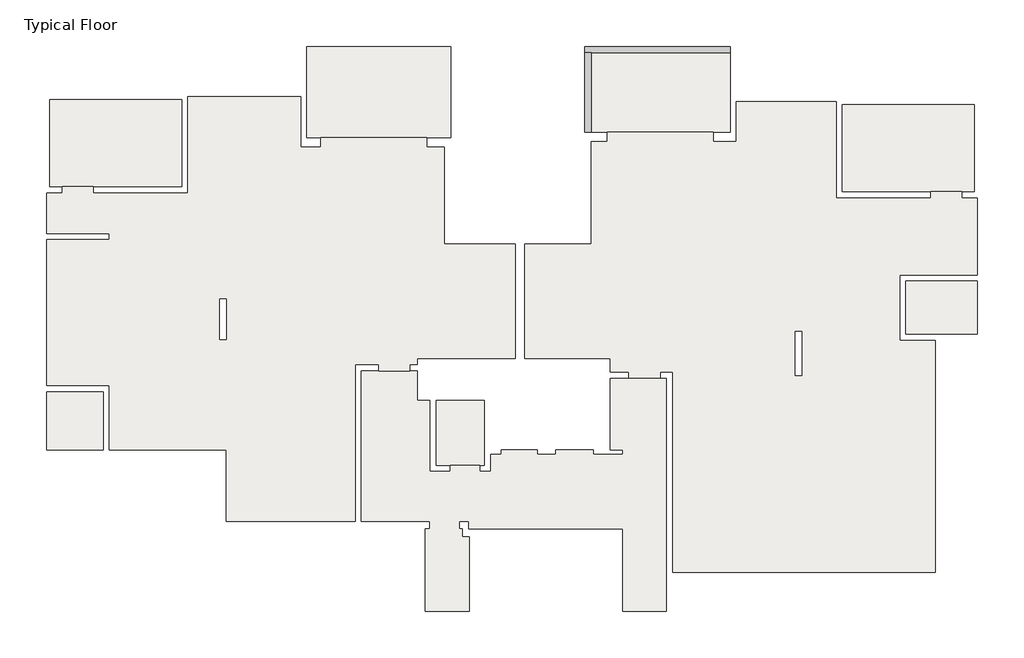
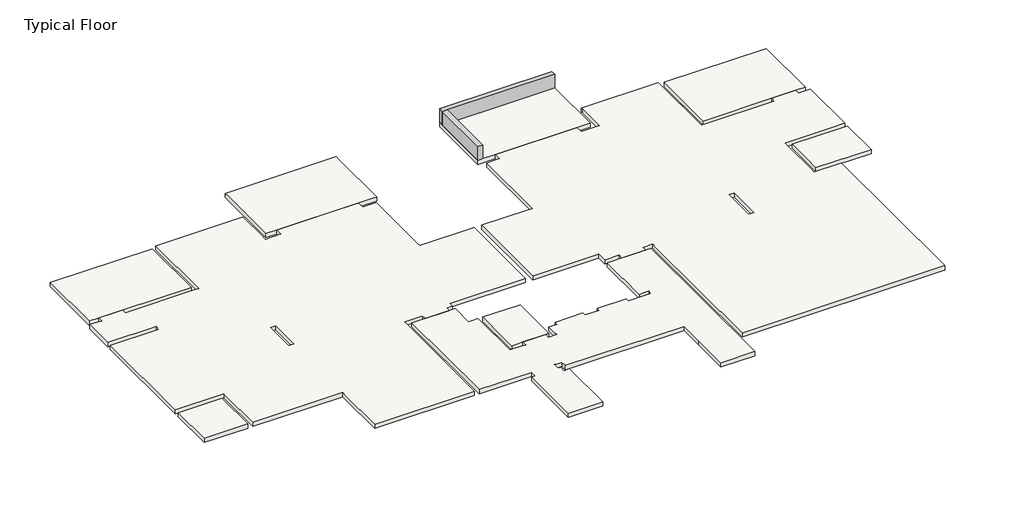
# One storey: 10 slabs, 2 beams.
"""IFC4 building model written with IfcOpenShell, lengths in millimetres."""

from ifc_helpers import new_model, si_unit, frame, origin, place, context, project, spatial, polyline, outline, extrude, faceted_brep, element, save

model = new_model("IFC4")

# Units and contexts
model_context = context("Model", 3, world=origin())
ifc_project = project(units=[si_unit("LENGTHUNIT", "METRE", prefix="MILLI")], contexts=[model_context])

# Site, building, storey
site = spatial("IfcSite", under=ifc_project)
building = spatial("IfcBuilding", under=site)
storey = spatial("IfcBuildingStorey", under=building, Name="Typical Floor", Elevation=3100.0)

# Beams
placement = place(None, origin())
element("IfcBeam", 1, ObjectType="Concrete Rectengular Beam : 20/60", at=placement, inside=storey, context=model_context, shape_type="Brep", body=[
    faceted_brep([(-2122.7212244, 19547.6197125, 3100.0), (-2122.7212244, 19547.6197125, 3700.0), (-2122.7212244, 19347.6197125, 3700.0), (-2122.7212244, 19347.6197125, 3100.0), (-6772.4580665, 19547.6197125, 3700.0), (-6772.4580665, 19347.6197125, 3700.0), (-6572.4580665, 19347.6197125, 3700.0), (-6772.4580665, 19347.6197125, 3100.0), (-6572.4580665, 19347.6197125, 3100.0), (-6772.4580665, 19547.6197125, 3100.0)], [[[0, 1, 2, 3]], [[2, 1, 4, 5, 6]], [[3, 2, 6, 5, 7, 8]], [[0, 3, 8, 7, 9]], [[1, 0, 9, 4]], [[5, 4, 9, 7]]]),
])
element("IfcBeam", 2, ObjectType="Concrete Rectengular Beam : 20/60", at=placement, inside=storey, context=model_context, shape_type="SweptSolid", body=[
    extrude(outline(polyline([(-6572.4580665, 16800.2512915), (-6772.4580665, 16800.2512915), (-6772.4580665, 19347.6197125), (-6572.4580665, 19347.6197125), (-6572.4580665, 16800.2512915)])), frame((0.0, 0.0, 3100.0), z_axis=(0.0, 0.0, 1.0), x_axis=(1.0, 0.0, 0.0)), (0.0, 0.0, 1.0), 600.0),
])

# Slabs
element("IfcSlab", 3, ObjectType="18", at=placement, inside=storey, context=model_context, shape_type="Brep", body=[
    faceted_brep([(-19660.8791191, 17843.4091862, 2920.0), (-19660.8791191, 15061.303923, 2920.0), (-22490.8791191, 15061.303923, 2920.0), (-23484.0370138, 15061.303923, 2920.0), (-23878.7738559, 15061.303923, 2920.0), (-23878.7738559, 17843.4091862, 2920.0), (-19660.8791191, 17843.4091862, 3100.0), (-23878.7738559, 17843.4091862, 3100.0), (-23878.7738559, 15061.303923, 3100.0), (-23484.0370138, 15061.303923, 3100.0), (-22490.8791191, 15061.303923, 3100.0), (-19660.8791191, 15061.303923, 3100.0)], [[[0, 1, 2, 3, 4, 5]], [[6, 7, 8, 9, 10, 11]], [[1, 0, 6, 11]], [[4, 3, 2, 1, 11, 10, 9, 8]], [[5, 4, 8, 7]], [[0, 5, 7, 6]]]),
])
element("IfcSlab", 4, ObjectType="18", at=placement, inside=storey, context=model_context, shape_type="SweptSolid", body=[
    extrude(outline(polyline([(-22170.3528033, 8497.0933967), (-22170.3528033, 6638.1460283), (-23980.8791191, 6638.1460283), (-23980.8791191, 8497.0933967), (-22170.3528033, 8497.0933967)])), frame((0.0, 0.0, 2920.0), z_axis=(0.0, 0.0, 1.0), x_axis=(1.0, 0.0, 0.0)), (0.0, 0.0, 1.0), 180.0),
])
element("IfcSlab", 5, ObjectType="18", at=placement, inside=storey, context=model_context, shape_type="SweptSolid", body=[
    extrude(outline(polyline([(5781.2261441, 12041.303923), (5781.2261441, 10343.4091862), (3494.9103546, 10343.4091862), (3494.9103546, 12041.303923), (5781.2261441, 12041.303923)])), frame((0.0, 0.0, 2920.0), z_axis=(0.0, 0.0, 1.0), x_axis=(1.0, 0.0, 0.0)), (0.0, 0.0, 1.0), 180.0),
])
element("IfcSlab", 6, ObjectType="18", at=placement, inside=storey, context=model_context, shape_type="Brep", body=[
    faceted_brep([(5680.1735125, 17683.4091862, 2920.0), (5680.1735125, 14901.303923, 2920.0), (5285.4366704, 14901.303923, 2920.0), (4292.2787756, 14901.303923, 2920.0), (1462.2787756, 14901.303923, 2920.0), (1462.2787756, 17683.4091862, 2920.0), (5680.1735125, 17683.4091862, 3100.0), (1462.2787756, 17683.4091862, 3100.0), (1462.2787756, 14901.303923, 3100.0), (4292.2787756, 14901.303923, 3100.0), (5285.4366704, 14901.303923, 3100.0), (5680.1735125, 14901.303923, 3100.0)], [[[0, 1, 2, 3, 4, 5]], [[6, 7, 8, 9, 10, 11]], [[1, 0, 6, 11]], [[4, 3, 2, 1, 11, 10, 9, 8]], [[5, 4, 8, 7]], [[0, 5, 7, 6]]]),
])
element("IfcSlab", 7, ObjectType="18", at=placement, inside=storey, context=model_context, shape_type="Brep", body=[
    faceted_brep([(-2122.7212244, 19547.6197125, 2920.0), (-2122.7212244, 16800.2512915, 2920.0), (-2672.7212244, 16800.2512915, 2920.0), (-6057.4580665, 16800.2512915, 2920.0), (-6772.4580665, 16800.2512915, 2920.0), (-6772.4580665, 19547.6197125, 2920.0), (-2122.7212244, 19547.6197125, 3100.0), (-6772.4580665, 19547.6197125, 3100.0), (-6772.4580665, 19347.6197125, 3100.0), (-6772.4580665, 16800.2512915, 3100.0), (-6572.4580665, 16800.2512915, 3100.0), (-6057.4580665, 16800.2512915, 3100.0), (-2672.7212244, 16800.2512915, 3100.0), (-2122.7212244, 16800.2512915, 3100.0), (-2122.7212244, 19347.6197125, 3100.0), (-2122.7212244, 19545.5144494, 3100.0)], [[[0, 1, 2, 3, 4, 5]], [[6, 7, 8, 9, 10, 11, 12, 13, 14, 15]], [[1, 0, 6, 15, 14, 13]], [[4, 3, 2, 1, 13, 12, 11, 10, 9]], [[5, 4, 9, 8, 7]], [[0, 5, 7, 6]]]),
])
element("IfcSlab", 8, ObjectType="18", at=placement, inside=storey, context=model_context, shape_type="Brep", body=[
    faceted_brep([(-15654.5633296, 19547.6197125, 2920.0), (-11058.7738559, 19547.6197125, 2920.0), (-11058.7738559, 16632.8828704, 2920.0), (-11825.0896454, 16632.8828704, 2920.0), (-15208.2475402, 16632.8828704, 2920.0), (-15654.5633296, 16632.8828704, 2920.0), (-15654.5633296, 19547.6197125, 3100.0), (-15654.5633296, 19545.5144494, 3100.0), (-15654.5633296, 19347.6197125, 3100.0), (-15654.5633296, 16632.8828704, 3100.0), (-15208.2475402, 16632.8828704, 3100.0), (-11825.0896454, 16632.8828704, 3100.0), (-11258.7738559, 16632.8828704, 3100.0), (-11058.7738559, 16632.8828704, 3100.0), (-11058.7738559, 19347.6197125, 3100.0), (-11058.7738559, 19547.6197125, 3100.0)], [[[0, 1, 2, 3, 4, 5]], [[6, 7, 8, 9, 10, 11, 12, 13, 14, 15]], [[1, 0, 6, 15]], [[2, 1, 15, 14, 13]], [[5, 4, 3, 2, 13, 12, 11, 10, 9]], [[0, 5, 9, 8, 7, 6]]]),
])
element("IfcSlab", 9, ObjectType="18", at=placement, inside=storey, context=model_context, shape_type="Brep", body=[
    faceted_brep([(-23980.8791191, 14861.303923, 2920.0), (-23484.0370138, 14861.303923, 2920.0), (-23484.0370138, 15061.303923, 2920.0), (-22490.8791191, 15061.303923, 2920.0), (-22490.8791191, 14861.303923, 2920.0), (-19660.8791191, 14861.303923, 2920.0), (-19460.8791191, 14861.303923, 2920.0), (-19460.8791191, 17943.4091862, 2920.0), (-15854.5633296, 17943.4091862, 2920.0), (-15854.5633296, 16632.8828704, 2920.0), (-15854.5633296, 16332.8828704, 2920.0), (-15208.2475402, 16332.8828704, 2920.0), (-15208.2475402, 16632.8828704, 2920.0), (-11825.0896454, 16632.8828704, 2920.0), (-11825.0896454, 16332.8828704, 2920.0), (-11258.7738559, 16332.8828704, 2920.0), (-11258.7738559, 13421.303923, 2920.0), (-11258.7738559, 13221.303923, 2920.0), (-8991.4054349, 13221.303923, 2920.0), (-8991.4054349, 9562.3565546, 2920.0), (-12124.0370138, 9562.3565546, 2920.0), (-12124.0370138, 9370.9220034, 2920.0), (-12364.0370138, 9370.9220034, 2920.0), (-12364.0370138, 9170.9220034, 2920.0), (-13360.7601979, 9170.9220034, 2920.0), (-13360.7601979, 9370.9220034, 2920.0), (-14113.5106981, 9370.9220034, 2920.0), (-14113.5106981, 9170.9220034, 2920.0), (-14113.5106981, 4357.6197125, 2920.0), (-18241.9317507, 4357.6197125, 2920.0), (-18241.9317507, 6438.1460283, 2920.0), (-18241.9317507, 6638.1460283, 2920.0), (-21970.3528033, 6638.1460283, 2920.0), (-21970.3528033, 8497.0933967, 2920.0), (-21970.3528033, 8697.0933967, 2920.0), (-23980.8791191, 8697.0933967, 2920.0), (-23980.8791191, 13368.6723441, 2920.0), (-21970.3528033, 13368.6723441, 2920.0), (-21970.3528033, 13568.6723441, 2920.0), (-23980.8791191, 13568.6723441, 2920.0), (-18235.4928274, 11466.5670809, 2920.0), (-18435.4928274, 11466.5670809, 2920.0), (-18435.4928274, 10166.5670809, 2920.0), (-18235.4928274, 10166.5670809, 2920.0), (-23484.0370138, 14861.303923, 3100.0), (-23980.8791191, 14861.303923, 3100.0), (-23980.8791191, 13568.6723441, 3100.0), (-21970.3528033, 13568.6723441, 3100.0), (-21970.3528033, 13368.6723441, 3100.0), (-23980.8791191, 13368.6723441, 3100.0), (-23980.8791191, 8697.0933967, 3100.0), (-21970.3528033, 8697.0933967, 3100.0), (-21970.3528033, 8497.0933967, 3100.0), (-21970.3528033, 6638.1460283, 3100.0), (-18241.9317507, 6638.1460283, 3100.0), (-18241.9317507, 6438.1460283, 3100.0), (-18241.9317507, 4357.6197125, 3100.0), (-14113.5106981, 4357.6197125, 3100.0), (-14113.5106981, 9170.9220034, 3100.0), (-14113.5106981, 9370.9220034, 3100.0), (-13360.7601979, 9370.9220034, 3100.0), (-13360.7601979, 9170.9220034, 3100.0), (-12364.0370138, 9170.9220034, 3100.0), (-12364.0370138, 9370.9220034, 3100.0), (-12124.0370138, 9370.9220034, 3100.0), (-12124.0370138, 9562.3565546, 3100.0), (-8991.4054349, 9562.3565546, 3100.0), (-8991.4054349, 13221.303923, 3100.0), (-11258.7738559, 13221.303923, 3100.0), (-11258.7738559, 13421.303923, 3100.0), (-11258.7738559, 16332.8828704, 3100.0), (-11825.0896454, 16332.8828704, 3100.0), (-11825.0896454, 16632.8828704, 3100.0), (-15208.2475402, 16632.8828704, 3100.0), (-15208.2475402, 16332.8828704, 3100.0), (-15854.5633296, 16332.8828704, 3100.0), (-15854.5633296, 16632.8828704, 3100.0), (-15854.5633296, 17943.4091862, 3100.0), (-19460.8791191, 17943.4091862, 3100.0), (-19460.8791191, 14861.303923, 3100.0), (-19660.8791191, 14861.303923, 3100.0), (-22490.8791191, 14861.303923, 3100.0), (-22490.8791191, 15061.303923, 3100.0), (-23484.0370138, 15061.303923, 3100.0), (-18435.4928274, 11466.5670809, 3100.0), (-18235.4928274, 11466.5670809, 3100.0), (-18235.4928274, 10166.5670809, 3100.0), (-18435.4928274, 10166.5670809, 3100.0)], [[[0, 1, 2, 3, 4, 5, 6, 7, 8, 9, 10, 11, 12, 13, 14, 15, 16, 17, 18, 19, 20, 21, 22, 23, 24, 25, 26, 27, 28, 29, 30, 31, 32, 33, 34, 35, 36, 37, 38, 39], [40, 41, 42, 43]], [[44, 45, 46, 47, 48, 49, 50, 51, 52, 53, 54, 55, 56, 57, 58, 59, 60, 61, 62, 63, 64, 65, 66, 67, 68, 69, 70, 71, 72, 73, 74, 75, 76, 77, 78, 79, 80, 81, 82, 83], [84, 85, 86, 87]], [[1, 0, 45, 44]], [[2, 1, 44, 83]], [[3, 2, 83, 82]], [[4, 3, 82, 81]], [[4, 81, 80, 79, 6, 5]], [[7, 6, 79, 78]], [[8, 7, 78, 77]], [[8, 77, 76, 75, 10, 9]], [[11, 10, 75, 74]], [[12, 11, 74, 73]], [[13, 12, 73, 72]], [[14, 13, 72, 71]], [[15, 14, 71, 70]], [[15, 70, 69, 68, 17, 16]], [[18, 17, 68, 67]], [[19, 18, 67, 66]], [[20, 19, 66, 65]], [[21, 20, 65, 64]], [[22, 21, 64, 63]], [[23, 22, 63, 62]], [[24, 23, 62, 61]], [[25, 24, 61, 60]], [[26, 25, 60, 59]], [[26, 59, 58, 57, 28, 27]], [[29, 28, 57, 56]], [[29, 56, 55, 54, 31, 30]], [[32, 31, 54, 53]], [[32, 53, 52, 51, 34, 33]], [[35, 34, 51, 50]], [[36, 35, 50, 49]], [[37, 36, 49, 48]], [[38, 37, 48, 47]], [[39, 38, 47, 46]], [[0, 39, 46, 45]], [[41, 40, 85, 84]], [[42, 41, 84, 87]], [[43, 42, 87, 86]], [[40, 43, 86, 85]]]),
])
element("IfcSlab", 10, ObjectType="18", at=placement, inside=storey, context=model_context, shape_type="Brep", body=[
    faceted_brep([(-6572.4580665, 13221.303923, 2920.0), (-6572.4580665, 16500.2512915, 2920.0), (-6057.4580665, 16500.2512915, 2920.0), (-6057.4580665, 16800.2512915, 2920.0), (-2672.7212244, 16800.2512915, 2920.0), (-2672.7212244, 16500.2512915, 2920.0), (-1922.7212244, 16500.2512915, 2920.0), (-1922.7212244, 16800.2512915, 2920.0), (-1922.7212244, 17700.2512915, 2920.0), (-1922.7212244, 17783.4091862, 2920.0), (1262.2787756, 17783.4091862, 2920.0), (1262.2787756, 14701.303923, 2920.0), (1462.2787756, 14701.303923, 2920.0), (4292.2787756, 14701.303923, 2920.0), (4292.2787756, 14901.303923, 2920.0), (5285.4366704, 14901.303923, 2920.0), (5285.4366704, 14701.303923, 2920.0), (5782.2787756, 14701.303923, 2920.0), (5782.2787756, 12241.303923, 2920.0), (3294.9103546, 12241.303923, 2920.0), (3294.9103546, 12041.303923, 2920.0), (3294.9103546, 10343.4091862, 2920.0), (3294.9103546, 10143.4091862, 2920.0), (4435.9629862, 10143.4091862, 2920.0), (4435.9629862, 2716.0407652, 2920.0), (-3966.142277, 2716.0407652, 2920.0), (-3966.142277, 8930.7776073, 2920.0), (-3966.142277, 9130.7776073, 2920.0), (-4366.142277, 9130.7776073, 2920.0), (-4366.142277, 8930.7776073, 2920.0), (-5359.8264875, 8930.7776073, 2920.0), (-5359.8264875, 9130.7776073, 2920.0), (-5957.7212244, 9130.7776073, 2920.0), (-5957.7212244, 9312.3565546, 2920.0), (-5957.7212244, 9562.3565546, 2920.0), (-8691.4054349, 9562.3565546, 2920.0), (-8691.4054349, 13221.303923, 2920.0), (-6772.4580665, 13221.303923, 2920.0), (-37.7212244, 10426.8302388, 2920.0), (-37.7212244, 9026.8302388, 2920.0), (162.2787756, 9026.8302388, 2920.0), (162.2787756, 10426.8302388, 2920.0), (-6572.4580665, 16500.2512915, 3100.0), (-6572.4580665, 13221.303923, 3100.0), (-6772.4580665, 13221.303923, 3100.0), (-8691.4054349, 13221.303923, 3100.0), (-8691.4054349, 9562.3565546, 3100.0), (-5957.7212244, 9562.3565546, 3100.0), (-5957.7212244, 9312.3565546, 3100.0), (-5957.7212244, 9130.7776073, 3100.0), (-5359.8264875, 9130.7776073, 3100.0), (-5359.8264875, 8930.7776073, 3100.0), (-4366.142277, 8930.7776073, 3100.0), (-4366.142277, 9130.7776073, 3100.0), (-3966.142277, 9130.7776073, 3100.0), (-3966.142277, 8930.7776073, 3100.0), (-3966.142277, 2716.0407652, 3100.0), (4435.9629862, 2716.0407652, 3100.0), (4435.9629862, 10143.4091862, 3100.0), (3294.9103546, 10143.4091862, 3100.0), (3294.9103546, 10343.4091862, 3100.0), (3294.9103546, 12041.303923, 3100.0), (3294.9103546, 12241.303923, 3100.0), (5782.2787756, 12241.303923, 3100.0), (5782.2787756, 14701.303923, 3100.0), (5285.4366704, 14701.303923, 3100.0), (5285.4366704, 14901.303923, 3100.0), (4292.2787756, 14901.303923, 3100.0), (4292.2787756, 14701.303923, 3100.0), (1462.2787756, 14701.303923, 3100.0), (1262.2787756, 14701.303923, 3100.0), (1262.2787756, 17783.4091862, 3100.0), (-1922.7212244, 17783.4091862, 3100.0), (-1922.7212244, 17700.2512915, 3100.0), (-1922.7212244, 16800.2512915, 3100.0), (-1922.7212244, 16500.2512915, 3100.0), (-2672.7212244, 16500.2512915, 3100.0), (-2672.7212244, 16800.2512915, 3100.0), (-6057.4580665, 16800.2512915, 3100.0), (-6057.4580665, 16500.2512915, 3100.0), (-37.7212244, 9026.8302388, 3100.0), (-37.7212244, 10426.8302388, 3100.0), (162.2787756, 10426.8302388, 3100.0), (162.2787756, 9026.8302388, 3100.0)], [[[0, 1, 2, 3, 4, 5, 6, 7, 8, 9, 10, 11, 12, 13, 14, 15, 16, 17, 18, 19, 20, 21, 22, 23, 24, 25, 26, 27, 28, 29, 30, 31, 32, 33, 34, 35, 36, 37], [38, 39, 40, 41]], [[42, 43, 44, 45, 46, 47, 48, 49, 50, 51, 52, 53, 54, 55, 56, 57, 58, 59, 60, 61, 62, 63, 64, 65, 66, 67, 68, 69, 70, 71, 72, 73, 74, 75, 76, 77, 78, 79], [80, 81, 82, 83]], [[43, 0, 37, 36, 45, 44]], [[1, 0, 43, 42]], [[2, 1, 42, 79]], [[3, 2, 79, 78]], [[4, 3, 78, 77]], [[5, 4, 77, 76]], [[6, 5, 76, 75]], [[6, 75, 74, 73, 8, 7]], [[9, 8, 73, 72]], [[10, 9, 72, 71]], [[11, 10, 71, 70]], [[11, 70, 69, 68, 13, 12]], [[14, 13, 68, 67]], [[15, 14, 67, 66]], [[16, 15, 66, 65]], [[17, 16, 65, 64]], [[18, 17, 64, 63]], [[19, 18, 63, 62]], [[19, 62, 61, 60, 59, 22, 21, 20]], [[23, 22, 59, 58]], [[24, 23, 58, 57]], [[25, 24, 57, 56]], [[25, 56, 55, 54, 27, 26]], [[28, 27, 54, 53]], [[29, 28, 53, 52]], [[30, 29, 52, 51]], [[31, 30, 51, 50]], [[32, 31, 50, 49]], [[32, 49, 48, 47, 34, 33]], [[35, 34, 47, 46]], [[36, 35, 46, 45]], [[39, 38, 81, 80]], [[40, 39, 80, 83]], [[41, 40, 83, 82]], [[38, 41, 82, 81]]]),
])
element("IfcSlab", 11, ObjectType="18", at=placement, inside=storey, context=model_context, shape_type="Brep", body=[
    faceted_brep([(-11726.142277, 8219.1986599, 2920.0), (-11726.142277, 5947.6197125, 2920.0), (-11526.142277, 5947.6197125, 2920.0), (-11069.3001717, 5947.6197125, 2920.0), (-11069.3001717, 6147.6197125, 2920.0), (-10124.0370138, 6147.6197125, 2920.0), (-10124.0370138, 5947.6197125, 2920.0), (-9785.0896454, 5947.6197125, 2920.0), (-9785.0896454, 6147.6197125, 2920.0), (-9785.0896454, 6494.4618178, 2920.0), (-9437.7212244, 6494.4618178, 2920.0), (-9437.7212244, 6644.4618178, 2920.0), (-8294.5633296, 6644.4618178, 2920.0), (-8294.5633296, 6494.4618178, 2920.0), (-7696.6685928, 6494.4618178, 2920.0), (-7696.6685928, 6644.4618178, 2920.0), (-6502.9843823, 6644.4618178, 2920.0), (-6502.9843823, 6494.9881336, 2920.0), (-5557.7212244, 6494.9881336, 2920.0), (-5557.7212244, 6644.9881336, 2920.0), (-5957.7212244, 6644.9881336, 2920.0), (-5957.7212244, 8930.7776073, 2920.0), (-5359.8264875, 8930.7776073, 2920.0), (-4366.142277, 8930.7776073, 2920.0), (-4166.142277, 8930.7776073, 2920.0), (-4166.142277, 1473.4091862, 2920.0), (-5559.8264875, 1473.4091862, 2920.0), (-5559.8264875, 2094.9881336, 2920.0), (-5559.8264875, 2591.8302388, 2920.0), (-5559.8264875, 3063.4091862, 2920.0), (-5559.8264875, 3859.1986599, 2920.0), (-5559.8264875, 4109.1986599, 2920.0), (-10481.9317507, 4109.1986599, 2920.0), (-10481.9317507, 4358.1460283, 2920.0), (-10681.9317507, 4358.1460283, 2920.0), (-10791.4054349, 4358.1460283, 2920.0), (-10791.4054349, 4108.1460283, 2920.0), (-10681.9317507, 4108.1460283, 2920.0), (-10681.9317507, 3859.1986599, 2920.0), (-10481.9317507, 3859.1986599, 2920.0), (-10462.9843823, 3859.1986599, 2920.0), (-10462.9843823, 1473.4091862, 2920.0), (-11875.6159612, 1473.4091862, 2920.0), (-11875.6159612, 4107.6197125, 2920.0), (-11736.6685928, 4107.6197125, 2920.0), (-11736.6685928, 4357.6197125, 2920.0), (-13913.5106981, 4357.6197125, 2920.0), (-13913.5106981, 9170.9220034, 2920.0), (-13360.7601979, 9170.9220034, 2920.0), (-12364.0370138, 9170.9220034, 2920.0), (-12124.0370138, 9170.9220034, 2920.0), (-12124.0370138, 8219.1986599, 2920.0), (-11874.0370138, 8219.1986599, 2920.0), (-11726.142277, 5947.6197125, 3100.0), (-11726.142277, 8219.1986599, 3100.0), (-11874.0370138, 8219.1986599, 3100.0), (-12124.0370138, 8219.1986599, 3100.0), (-12124.0370138, 9170.9220034, 3100.0), (-12364.0370138, 9170.9220034, 3100.0), (-13360.7601979, 9170.9220034, 3100.0), (-13913.5106981, 9170.9220034, 3100.0), (-13913.5106981, 4357.6197125, 3100.0), (-11736.6685928, 4357.6197125, 3100.0), (-11736.6685928, 4107.6197125, 3100.0), (-11875.6159612, 4107.6197125, 3100.0), (-11875.6159612, 1473.4091862, 3100.0), (-10462.9843823, 1473.4091862, 3100.0), (-10462.9843823, 3859.1986599, 3100.0), (-10481.9317507, 3859.1986599, 3100.0), (-10681.9317507, 3859.1986599, 3100.0), (-10681.9317507, 4108.1460283, 3100.0), (-10791.4054349, 4108.1460283, 3100.0), (-10791.4054349, 4358.1460283, 3100.0), (-10681.9317507, 4358.1460283, 3100.0), (-10481.9317507, 4358.1460283, 3100.0), (-10481.9317507, 4109.1986599, 3100.0), (-5559.8264875, 4109.1986599, 3100.0), (-5559.8264875, 3859.1986599, 3100.0), (-5559.8264875, 3063.4091862, 3100.0), (-5559.8264875, 2591.8302388, 3100.0), (-5559.8264875, 2094.9881336, 3100.0), (-5559.8264875, 1473.4091862, 3100.0), (-4166.142277, 1473.4091862, 3100.0), (-4166.142277, 8930.7776073, 3100.0), (-4366.142277, 8930.7776073, 3100.0), (-5359.8264875, 8930.7776073, 3100.0), (-5957.7212244, 8930.7776073, 3100.0), (-5957.7212244, 6644.9881336, 3100.0), (-5557.7212244, 6644.9881336, 3100.0), (-5557.7212244, 6494.9881336, 3100.0), (-6502.9843823, 6494.9881336, 3100.0), (-6502.9843823, 6644.4618178, 3100.0), (-7696.6685928, 6644.4618178, 3100.0), (-7696.6685928, 6494.4618178, 3100.0), (-8294.5633296, 6494.4618178, 3100.0), (-8294.5633296, 6644.4618178, 3100.0), (-9437.7212244, 6644.4618178, 3100.0), (-9437.7212244, 6494.4618178, 3100.0), (-9785.0896454, 6494.4618178, 3100.0), (-9785.0896454, 6147.6197125, 3100.0), (-9785.0896454, 5947.6197125, 3100.0), (-10124.0370138, 5947.6197125, 3100.0), (-10124.0370138, 6147.6197125, 3100.0), (-11069.3001717, 6147.6197125, 3100.0), (-11069.3001717, 5947.6197125, 3100.0), (-11526.142277, 5947.6197125, 3100.0)], [[[0, 1, 2, 3, 4, 5, 6, 7, 8, 9, 10, 11, 12, 13, 14, 15, 16, 17, 18, 19, 20, 21, 22, 23, 24, 25, 26, 27, 28, 29, 30, 31, 32, 33, 34, 35, 36, 37, 38, 39, 40, 41, 42, 43, 44, 45, 46, 47, 48, 49, 50, 51, 52]], [[53, 54, 55, 56, 57, 58, 59, 60, 61, 62, 63, 64, 65, 66, 67, 68, 69, 70, 71, 72, 73, 74, 75, 76, 77, 78, 79, 80, 81, 82, 83, 84, 85, 86, 87, 88, 89, 90, 91, 92, 93, 94, 95, 96, 97, 98, 99, 100, 101, 102, 103, 104, 105]], [[56, 51, 50, 57]], [[51, 56, 55, 54, 0, 52]], [[1, 0, 54, 53]], [[1, 53, 105, 104, 3, 2]], [[4, 3, 104, 103]], [[5, 4, 103, 102]], [[6, 5, 102, 101]], [[7, 6, 101, 100]], [[7, 100, 99, 98, 9, 8]], [[10, 9, 98, 97]], [[11, 10, 97, 96]], [[12, 11, 96, 95]], [[13, 12, 95, 94]], [[14, 13, 94, 93]], [[15, 14, 93, 92]], [[16, 15, 92, 91]], [[17, 16, 91, 90]], [[18, 17, 90, 89]], [[19, 18, 89, 88]], [[20, 19, 88, 87]], [[21, 20, 87, 86]], [[21, 86, 85, 84, 83, 24, 23, 22]], [[25, 24, 83, 82]], [[26, 25, 82, 81]], [[26, 81, 80, 79, 78, 29, 28, 27]], [[29, 78, 77, 76, 31, 30]], [[32, 31, 76, 75]], [[33, 32, 75, 74]], [[33, 74, 73, 72, 35, 34]], [[36, 35, 72, 71]], [[37, 36, 71, 70]], [[38, 37, 70, 69]], [[38, 69, 68, 67, 40, 39]], [[41, 40, 67, 66]], [[42, 41, 66, 65]], [[43, 42, 65, 64]], [[44, 43, 64, 63]], [[45, 44, 63, 62]], [[46, 45, 62, 61]], [[46, 61, 60, 47]], [[47, 60, 59, 58, 57, 50, 49, 48]]]),
])
element("IfcSlab", 12, ObjectType="18", at=placement, inside=storey, context=model_context, shape_type="Brep", body=[
    faceted_brep([(-9985.0896454, 8219.1986599, 2920.0), (-9985.0896454, 6147.6197125, 2920.0), (-10124.0370138, 6147.6197125, 2920.0), (-11069.3001717, 6147.6197125, 2920.0), (-11526.142277, 6147.6197125, 2920.0), (-11526.142277, 8219.1986599, 2920.0), (-9985.0896454, 6147.6197125, 3100.0), (-9985.0896454, 8219.1986599, 3100.0), (-11526.142277, 8219.1986599, 3100.0), (-11526.142277, 6147.6197125, 3100.0), (-11069.3001717, 6147.6197125, 3100.0), (-10124.0370138, 6147.6197125, 3100.0)], [[[0, 1, 2, 3, 4, 5]], [[6, 7, 8, 9, 10, 11]], [[1, 0, 7, 6]], [[1, 6, 11, 10, 9, 4, 3, 2]], [[5, 4, 9, 8]], [[0, 5, 8, 7]]]),
])

save(model, "model.ifc")

# Revit data of these elements
# Type "Concrete Rectengular Beam : 20/60"
#   Length [instance default] = 152.4 cm
#   b = 20 cm
#   h = 60 cm
#   Structural Material [instance default] = Concrete
#   Assembly Code = ""
# Type "18"
#   Function = 0
#   Layers, outside or top first: 18 cm "Concrete" (function 1)
# Element 1 (IfcBeam, "Concrete Rectengular Beam : 20/60")
#   Comments = ""
#   Mark = "B3"
#   SOFiSTiK_AMG_Comments = ""
#   SOFiSTiK_AMG_Scheduled = yes
#   SOFiSTiK_AMG_Adjusted = yes
#   Structural Material = Concrete
#   Phase Created = New Construction
#   Materials on its faces: "Concrete"
# Element 2 (IfcBeam, "Concrete Rectengular Beam : 20/60")
#   Comments = ""
#   Mark = "B4"
#   SOFiSTiK_AMG_Comments = ""
#   SOFiSTiK_AMG_Scheduled = yes
#   SOFiSTiK_AMG_Adjusted = yes
#   Structural Material = Concrete
#   Phase Created = New Construction
#   Materials on its faces: "Concrete"
# Element 3 (IfcSlab, "18")
#   Mark = "S1"
#   SOFiSTiK_AMG_Comments = ""
#   Height Offset From Level = 0 cm
#   built-in parameter 1001954 = 1
#   SOFiSTiK_AMG_Scheduled = yes
#   SOFiSTiK_AMG_Adjusted = yes
#   Phase Created = New Construction
#   Materials on its faces: "Concrete"
# Element 4 (IfcSlab, "18")
#   Mark = "S2"
#   SOFiSTiK_AMG_Comments = ""
#   Height Offset From Level = 0 cm
#   built-in parameter 1001954 = 1
#   SOFiSTiK_AMG_Scheduled = yes
#   SOFiSTiK_AMG_Adjusted = yes
#   Phase Created = New Construction
#   Materials on its faces: "Concrete"
# Element 5 (IfcSlab, "18")
#   Mark = "S3"
#   SOFiSTiK_AMG_Comments = ""
#   Height Offset From Level = 0 cm
#   built-in parameter 1001954 = 1
#   SOFiSTiK_AMG_Scheduled = yes
#   SOFiSTiK_AMG_Adjusted = yes
#   Phase Created = New Construction
#   Materials on its faces: "Concrete"
# Element 6 (IfcSlab, "18")
#   Mark = "S4"
#   SOFiSTiK_AMG_Comments = ""
#   Height Offset From Level = 0 cm
#   built-in parameter 1001954 = 1
#   SOFiSTiK_AMG_Scheduled = yes
#   SOFiSTiK_AMG_Adjusted = yes
#   Phase Created = New Construction
#   Materials on its faces: "Concrete"
# Element 7 (IfcSlab, "18")
#   Mark = "S5"
#   SOFiSTiK_AMG_Comments = ""
#   Height Offset From Level = 0 cm
#   built-in parameter 1001954 = 1
#   SOFiSTiK_AMG_Scheduled = yes
#   SOFiSTiK_AMG_Adjusted = yes
#   Phase Created = New Construction
#   Materials on its faces: "Concrete"
# Element 8 (IfcSlab, "18")
#   Mark = "S6"
#   SOFiSTiK_AMG_Comments = ""
#   built-in parameter 1001955 = 3.14159 (stored number, unit not read)
#   Height Offset From Level = 0 cm
#   built-in parameter 1001954 = 1
#   SOFiSTiK_AMG_Scheduled = yes
#   SOFiSTiK_AMG_Adjusted = yes
#   Phase Created = New Construction
#   Materials on its faces: "Concrete"
# Element 9 (IfcSlab, "18")
#   Mark = "S7"
#   SOFiSTiK_AMG_Comments = ""
#   built-in parameter 1001955 = 1.5708 (stored number, unit not read)
#   Height Offset From Level = 0 cm
#   built-in parameter 1001954 = 1
#   SOFiSTiK_AMG_Scheduled = yes
#   SOFiSTiK_AMG_Adjusted = yes
#   Phase Created = New Construction
#   Materials on its faces: "Concrete"
# Element 10 (IfcSlab, "18")
#   Mark = "S8"
#   SOFiSTiK_AMG_Comments = ""
#   built-in parameter 1001955 = 1.5708 (stored number, unit not read)
#   Height Offset From Level = 0 cm
#   built-in parameter 1001954 = 1
#   SOFiSTiK_AMG_Scheduled = yes
#   SOFiSTiK_AMG_Adjusted = yes
#   Phase Created = New Construction
#   Materials on its faces: "Concrete"
# Element 11 (IfcSlab, "18")
#   Mark = "S9"
#   SOFiSTiK_AMG_Comments = ""
#   built-in parameter 1001955 = 1.5708 (stored number, unit not read)
#   Height Offset From Level = 0 cm
#   built-in parameter 1001954 = 1
#   SOFiSTiK_AMG_Scheduled = yes
#   SOFiSTiK_AMG_Adjusted = yes
#   Phase Created = New Construction
#   Materials on its faces: "Concrete"
# Element 12 (IfcSlab, "18")
#   Mark = "S10"
#   SOFiSTiK_AMG_Comments = ""
#   Height Offset From Level = 0 cm
#   built-in parameter 1001954 = 1
#   SOFiSTiK_AMG_Scheduled = yes
#   SOFiSTiK_AMG_Adjusted = yes
#   Phase Created = New Construction
#   Materials on its faces: "Concrete"
# Materials
#   "Concrete": class "Concrete", colour RGB 192 192 192, transparency 0, Keynote = "01000", Description = "Cast-in-place concrete", Cost = 0
